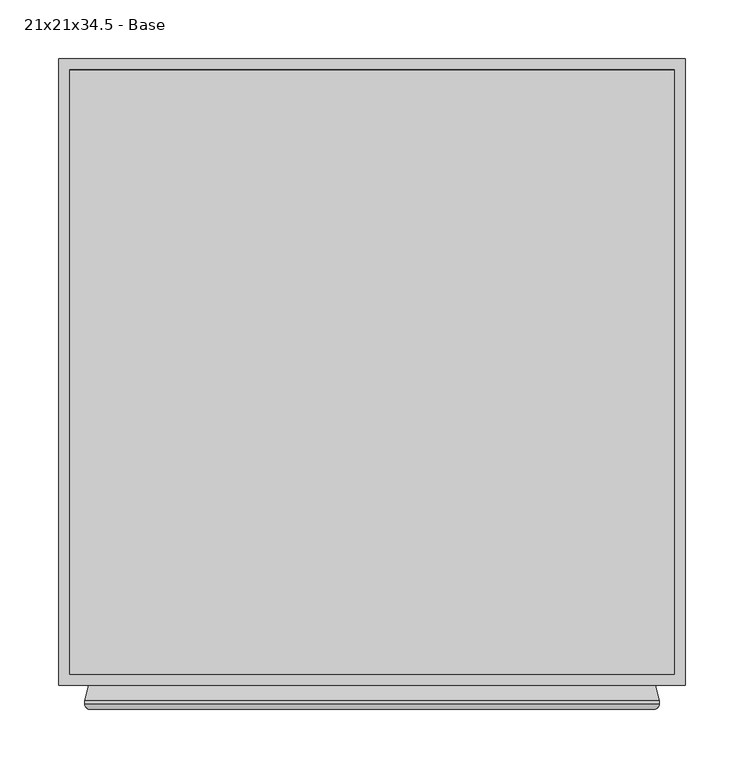
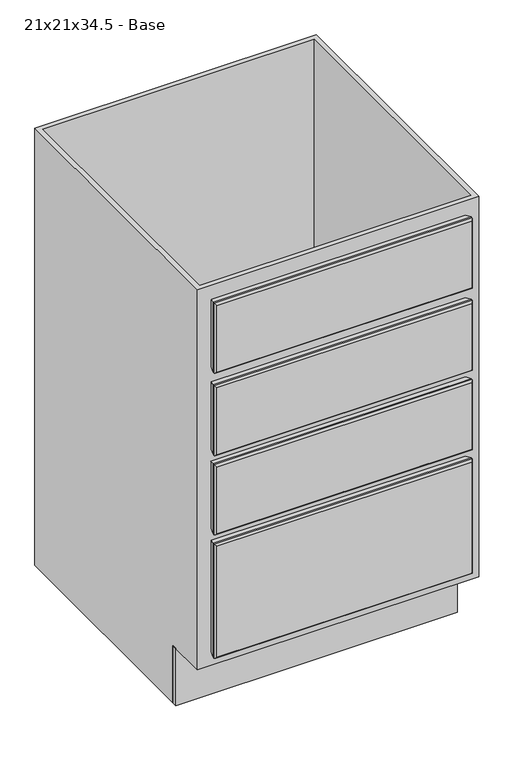
"""IFC4 building model written with IfcOpenShell, lengths in millimetres: furniture geometry, Cabinet-Base-Merillat-Four_Drawer-Marlin : 21x21x34.5 - Base."""

from ifc_helpers import new_model, si_unit, frame, origin, origin_with_axes, place, context, project, spatial, polyline, ellipse_curve, outline, extrude, faceted_brep, source, transform, mapped, element, save
from ifc_brep_helpers import plane_surface, cylinder_surface, advanced_brep


def furniture_21x21x34_5_base_fafdbe70(model_context):
    return source(origin(), model_context, "Body", "SolidModel", [
        advanced_brep(
        [(-222.6408026, -629.92, 365.2035075), (-222.6408026, -629.92, 142.7964925), (260.1162124, -629.92, 142.7964925), (260.1162124, -629.92, 365.2035075), (-222.2320951, -609.6, 143.2052), (-222.2320951, -609.6, 364.7948), (259.7075049, -609.6, 364.7948), (259.7075049, -609.6, 143.2052), (-225.7372951, -625.4496, 368.3), (-225.7372951, -622.681, 368.3), (-225.7372951, -622.681, 139.7), (-225.7372951, -625.4496, 139.7), (263.2127049, -622.681, 139.7), (263.2127049, -625.4496, 139.7), (263.2127049, -622.681, 368.3), (263.2127049, -625.4496, 368.3)],
        [
            (0, 1),
            (1, 2),
            (2, 3),
            (3, 0),
            (4, 5),
            (5, 6),
            (6, 7),
            (7, 4),
            (8, 9),
            (9, 10),
            (10, 11),
            (11, 8),
            (10, 12),
            (12, 13),
            (13, 11),
            (12, 14),
            (14, 15),
            (15, 13),
            (8, 15),
            (14, 9),
            (11, 1, ellipse_curve(frame((-220.9620951, -625.4496, 144.4752), z_axis=(-0.7071067811865475, 0.0, 0.7071067811865475), x_axis=(-0.7071067811865474, 0.0, -0.7071067811865476)), 6.7531526, 4.7752)),
            (0, 8, ellipse_curve(frame((-220.9620951, -625.4496, 363.5248), z_axis=(-0.7071067811865475, 0.0, -0.7071067811865475), x_axis=(0.7071067811865474, 0.0, -0.7071067811865476)), 6.7531526, 4.7752)),
            (4, 10),
            (9, 5),
            (13, 2, ellipse_curve(frame((258.4375049, -625.4496, 144.4752), z_axis=(-0.7071067811865475, 0.0, -0.7071067811865475), x_axis=(0.7071067811865476, 0.0, -0.7071067811865474)), 6.7531526, 4.7752)),
            (7, 12),
            (15, 3, ellipse_curve(frame((258.4375049, -625.4496, 363.5248), z_axis=(0.7071067811865475, 0.0, -0.7071067811865475), x_axis=(0.7071067811865474, 0.0, 0.7071067811865476)), 6.7531526, 4.7752)),
            (6, 14),
        ],
        [
            plane_surface(frame((-225.7372951, -629.92, 368.3), z_axis=(0.0, -1.0, 0.0), x_axis=(0.0, 0.0, -1.0))),
            plane_surface(frame((-225.7372951, -609.6, 368.3), z_axis=(0.0, 1.0, 0.0), x_axis=(0.0, 0.0, 1.0))),
            plane_surface(frame((-225.7372951, -629.92, 368.3), z_axis=(-1.0, 0.0, 0.0), x_axis=(0.0, 1.0, 0.0))),
            plane_surface(frame((-225.7372951, -629.92, 139.7), z_axis=(0.0, 0.0, -1.0), x_axis=(0.0, 1.0, 0.0))),
            plane_surface(frame((263.2127049, -629.92, 139.7), z_axis=(1.0, 0.0, 0.0), x_axis=(0.0, 1.0, 0.0))),
            plane_surface(frame((263.2127049, -629.92, 368.3), z_axis=(0.0, 0.0, 1.0), x_axis=(0.0, 1.0, 0.0))),
            cylinder_surface(frame((-220.9620951, -625.4496, 368.3), z_axis=(0.0, 0.0, -1.0), x_axis=(0.0, 1.0, 0.0)), 4.7752),
            plane_surface(frame((-225.7372951, -622.681, 368.3), z_axis=(-0.9659229350723619, 0.25882983502910506, 0.0), x_axis=(0.0, 0.0, -1.0))),
            cylinder_surface(frame((-225.7372951, -625.4496, 144.4752), z_axis=(1.0, 0.0, 0.0), x_axis=(0.0, 1.0, 0.0)), 4.7752),
            plane_surface(frame((-225.7372951, -622.681, 139.7), z_axis=(0.0, 0.25882983502910506, -0.9659229350723619), x_axis=(1.0, 0.0, 0.0))),
            cylinder_surface(frame((258.4375049, -625.4496, 139.7), z_axis=(0.0, 0.0, 1.0), x_axis=(0.0, 1.0, 0.0)), 4.7752),
            plane_surface(frame((263.2127049, -622.681, 139.7), z_axis=(0.9659229350723619, 0.25882983502910506, 0.0), x_axis=(0.0, 0.0, 1.0))),
            cylinder_surface(frame((263.2127049, -625.4496, 363.5248), z_axis=(-1.0, 0.0, 0.0), x_axis=(0.0, 1.0, 0.0)), 4.7752),
            plane_surface(frame((263.2127049, -622.681, 368.3), z_axis=(0.0, 0.25882983502910506, 0.9659229350723619), x_axis=(-1.0, 0.0, 0.0))),
        ],
        [
            (0, [[1, 2, 3, 4]]),
            (1, [[5, 6, 7, 8]]),
            (2, [[9, 10, 11, 12]]),
            (3, [[-11, 13, 14, 15]]),
            (4, [[-14, 16, 17, 18]]),
            (5, [[-9, 19, -17, 20]]),
            (6, [[21, -1, 22, -12]]),
            (7, [[23, -10, 24, -5]]),
            (8, [[-21, -15, 25, -2]]),
            (9, [[-23, -8, 26, -13]]),
            (10, [[-25, -18, 27, -3]]),
            (11, [[-26, -7, 28, -16]]),
            (12, [[-22, -4, -27, -19]]),
            (13, [[-24, -20, -28, -6]]),
        ],
    ),
        advanced_brep(
        [(-222.6408026, -629.92, 523.9535075), (-222.6408026, -629.92, 390.4464925), (260.1162124, -629.92, 390.4464925), (260.1162124, -629.92, 523.9535075), (-222.2320951, -609.6, 390.8552), (-222.2320951, -609.6, 523.5448), (259.7075049, -609.6, 523.5448), (259.7075049, -609.6, 390.8552), (-225.7372951, -625.4496, 527.05), (-225.7372951, -622.681, 527.05), (-225.7372951, -622.681, 387.35), (-225.7372951, -625.4496, 387.35), (263.2127049, -622.681, 387.35), (263.2127049, -625.4496, 387.35), (263.2127049, -622.681, 527.05), (263.2127049, -625.4496, 527.05)],
        [
            (0, 1),
            (1, 2),
            (2, 3),
            (3, 0),
            (4, 5),
            (5, 6),
            (6, 7),
            (7, 4),
            (8, 9),
            (9, 10),
            (10, 11),
            (11, 8),
            (10, 12),
            (12, 13),
            (13, 11),
            (12, 14),
            (14, 15),
            (15, 13),
            (8, 15),
            (14, 9),
            (11, 1, ellipse_curve(frame((-220.9620951, -625.4496, 392.1252), z_axis=(-0.7071067811865475, 0.0, 0.7071067811865475), x_axis=(-0.7071067811865474, 0.0, -0.7071067811865476)), 6.7531526, 4.7752)),
            (0, 8, ellipse_curve(frame((-220.9620951, -625.4496, 522.2748), z_axis=(-0.7071067811865475, 0.0, -0.7071067811865475), x_axis=(0.7071067811865474, 0.0, -0.7071067811865476)), 6.7531526, 4.7752)),
            (4, 10),
            (9, 5),
            (13, 2, ellipse_curve(frame((258.4375049, -625.4496, 392.1252), z_axis=(-0.7071067811865475, 0.0, -0.7071067811865475), x_axis=(0.7071067811865476, 0.0, -0.7071067811865474)), 6.7531526, 4.7752)),
            (7, 12),
            (15, 3, ellipse_curve(frame((258.4375049, -625.4496, 522.2748), z_axis=(0.7071067811865475, 0.0, -0.7071067811865475), x_axis=(0.7071067811865474, 0.0, 0.7071067811865476)), 6.7531526, 4.7752)),
            (6, 14),
        ],
        [
            plane_surface(frame((-225.7372951, -629.92, 527.05), z_axis=(0.0, -1.0, 0.0), x_axis=(0.0, 0.0, -1.0))),
            plane_surface(frame((-225.7372951, -609.6, 527.05), z_axis=(0.0, 1.0, 0.0), x_axis=(0.0, 0.0, 1.0))),
            plane_surface(frame((-225.7372951, -629.92, 527.05), z_axis=(-1.0, 0.0, 0.0), x_axis=(0.0, 1.0, 0.0))),
            plane_surface(frame((-225.7372951, -629.92, 387.35), z_axis=(0.0, 0.0, -1.0), x_axis=(0.0, 1.0, 0.0))),
            plane_surface(frame((263.2127049, -629.92, 387.35), z_axis=(1.0, 0.0, 0.0), x_axis=(0.0, 1.0, 0.0))),
            plane_surface(frame((263.2127049, -629.92, 527.05), z_axis=(0.0, 0.0, 1.0), x_axis=(0.0, 1.0, 0.0))),
            cylinder_surface(frame((-220.9620951, -625.4496, 527.05), z_axis=(0.0, 0.0, -1.0), x_axis=(0.0, 1.0, 0.0)), 4.7752),
            plane_surface(frame((-225.7372951, -622.681, 527.05), z_axis=(-0.9659229350723619, 0.25882983502910506, 0.0), x_axis=(0.0, 0.0, -1.0))),
            cylinder_surface(frame((-225.7372951, -625.4496, 392.1252), z_axis=(1.0, 0.0, 0.0), x_axis=(0.0, 1.0, 0.0)), 4.7752),
            plane_surface(frame((-225.7372951, -622.681, 387.35), z_axis=(0.0, 0.25882983502910506, -0.9659229350723619), x_axis=(1.0, 0.0, 0.0))),
            cylinder_surface(frame((258.4375049, -625.4496, 387.35), z_axis=(0.0, 0.0, 1.0), x_axis=(0.0, 1.0, 0.0)), 4.7752),
            plane_surface(frame((263.2127049, -622.681, 387.35), z_axis=(0.9659229350723619, 0.25882983502910506, 0.0), x_axis=(0.0, 0.0, 1.0))),
            cylinder_surface(frame((263.2127049, -625.4496, 522.2748), z_axis=(-1.0, 0.0, 0.0), x_axis=(0.0, 1.0, 0.0)), 4.7752),
            plane_surface(frame((263.2127049, -622.681, 527.05), z_axis=(0.0, 0.25882983502910506, 0.9659229350723619), x_axis=(-1.0, 0.0, 0.0))),
        ],
        [
            (0, [[1, 2, 3, 4]]),
            (1, [[5, 6, 7, 8]]),
            (2, [[9, 10, 11, 12]]),
            (3, [[-11, 13, 14, 15]]),
            (4, [[-14, 16, 17, 18]]),
            (5, [[-9, 19, -17, 20]]),
            (6, [[21, -1, 22, -12]]),
            (7, [[23, -10, 24, -5]]),
            (8, [[-21, -15, 25, -2]]),
            (9, [[-23, -8, 26, -13]]),
            (10, [[-25, -18, 27, -3]]),
            (11, [[-26, -7, 28, -16]]),
            (12, [[-22, -4, -27, -19]]),
            (13, [[-24, -20, -28, -6]]),
        ],
    ),
        advanced_brep(
        [(-222.6408026, -629.92, 682.7035075), (-222.6408026, -629.92, 549.1964925), (260.1162124, -629.92, 549.1964925), (260.1162124, -629.92, 682.7035075), (-222.2320951, -609.6, 549.6052), (-222.2320951, -609.6, 682.2948), (259.7075049, -609.6, 682.2948), (259.7075049, -609.6, 549.6052), (-225.7372951, -625.4496, 685.8), (-225.7372951, -622.681, 685.8), (-225.7372951, -622.681, 546.1), (-225.7372951, -625.4496, 546.1), (263.2127049, -622.681, 546.1), (263.2127049, -625.4496, 546.1), (263.2127049, -622.681, 685.8), (263.2127049, -625.4496, 685.8)],
        [
            (0, 1),
            (1, 2),
            (2, 3),
            (3, 0),
            (4, 5),
            (5, 6),
            (6, 7),
            (7, 4),
            (8, 9),
            (9, 10),
            (10, 11),
            (11, 8),
            (10, 12),
            (12, 13),
            (13, 11),
            (12, 14),
            (14, 15),
            (15, 13),
            (8, 15),
            (14, 9),
            (11, 1, ellipse_curve(frame((-220.9620951, -625.4496, 550.8752), z_axis=(-0.7071067811865475, 0.0, 0.7071067811865475), x_axis=(-0.7071067811865474, 0.0, -0.7071067811865476)), 6.7531526, 4.7752)),
            (0, 8, ellipse_curve(frame((-220.9620951, -625.4496, 681.0248), z_axis=(-0.7071067811865475, 0.0, -0.7071067811865475), x_axis=(0.7071067811865474, 0.0, -0.7071067811865476)), 6.7531526, 4.7752)),
            (4, 10),
            (9, 5),
            (13, 2, ellipse_curve(frame((258.4375049, -625.4496, 550.8752), z_axis=(-0.7071067811865475, 0.0, -0.7071067811865475), x_axis=(0.7071067811865476, 0.0, -0.7071067811865474)), 6.7531526, 4.7752)),
            (7, 12),
            (15, 3, ellipse_curve(frame((258.4375049, -625.4496, 681.0248), z_axis=(0.7071067811865475, 0.0, -0.7071067811865475), x_axis=(0.7071067811865474, 0.0, 0.7071067811865476)), 6.7531526, 4.7752)),
            (6, 14),
        ],
        [
            plane_surface(frame((-225.7372951, -629.92, 685.8), z_axis=(0.0, -1.0, 0.0), x_axis=(0.0, 0.0, -1.0))),
            plane_surface(frame((-225.7372951, -609.6, 685.8), z_axis=(0.0, 1.0, 0.0), x_axis=(0.0, 0.0, 1.0))),
            plane_surface(frame((-225.7372951, -629.92, 685.8), z_axis=(-1.0, 0.0, 0.0), x_axis=(0.0, 1.0, 0.0))),
            plane_surface(frame((-225.7372951, -629.92, 546.1), z_axis=(0.0, 0.0, -1.0), x_axis=(0.0, 1.0, 0.0))),
            plane_surface(frame((263.2127049, -629.92, 546.1), z_axis=(1.0, 0.0, 0.0), x_axis=(0.0, 1.0, 0.0))),
            plane_surface(frame((263.2127049, -629.92, 685.8), z_axis=(0.0, 0.0, 1.0), x_axis=(0.0, 1.0, 0.0))),
            cylinder_surface(frame((-220.9620951, -625.4496, 685.8), z_axis=(0.0, 0.0, -1.0), x_axis=(0.0, 1.0, 0.0)), 4.7752),
            plane_surface(frame((-225.7372951, -622.681, 685.8), z_axis=(-0.9659229350723619, 0.25882983502910506, 0.0), x_axis=(0.0, 0.0, -1.0))),
            cylinder_surface(frame((-225.7372951, -625.4496, 550.8752), z_axis=(1.0, 0.0, 0.0), x_axis=(0.0, 1.0, 0.0)), 4.7752),
            plane_surface(frame((-225.7372951, -622.681, 546.1), z_axis=(0.0, 0.25882983502910506, -0.9659229350723619), x_axis=(1.0, 0.0, 0.0))),
            cylinder_surface(frame((258.4375049, -625.4496, 546.1), z_axis=(0.0, 0.0, 1.0), x_axis=(0.0, 1.0, 0.0)), 4.7752),
            plane_surface(frame((263.2127049, -622.681, 546.1), z_axis=(0.9659229350723619, 0.25882983502910506, 0.0), x_axis=(0.0, 0.0, 1.0))),
            cylinder_surface(frame((263.2127049, -625.4496, 681.0248), z_axis=(-1.0, 0.0, 0.0), x_axis=(0.0, 1.0, 0.0)), 4.7752),
            plane_surface(frame((263.2127049, -622.681, 685.8), z_axis=(0.0, 0.25882983502910506, 0.9659229350723619), x_axis=(-1.0, 0.0, 0.0))),
        ],
        [
            (0, [[1, 2, 3, 4]]),
            (1, [[5, 6, 7, 8]]),
            (2, [[9, 10, 11, 12]]),
            (3, [[-11, 13, 14, 15]]),
            (4, [[-14, 16, 17, 18]]),
            (5, [[-9, 19, -17, 20]]),
            (6, [[21, -1, 22, -12]]),
            (7, [[23, -10, 24, -5]]),
            (8, [[-21, -15, 25, -2]]),
            (9, [[-23, -8, 26, -13]]),
            (10, [[-25, -18, 27, -3]]),
            (11, [[-26, -7, 28, -16]]),
            (12, [[-22, -4, -27, -19]]),
            (13, [[-24, -20, -28, -6]]),
        ],
    ),
        advanced_brep(
        [(-222.6408026, -629.92, 847.8035075), (-222.6408026, -629.92, 714.2964925), (260.1162124, -629.92, 714.2964925), (260.1162124, -629.92, 847.8035075), (-222.2320951, -609.6, 714.7052), (-222.2320951, -609.6, 847.3948), (259.7075049, -609.6, 847.3948), (259.7075049, -609.6, 714.7052), (-225.7372951, -625.4496, 850.9), (-225.7372951, -622.681, 850.9), (-225.7372951, -622.681, 711.2), (-225.7372951, -625.4496, 711.2), (263.2127049, -622.681, 711.2), (263.2127049, -625.4496, 711.2), (263.2127049, -622.681, 850.9), (263.2127049, -625.4496, 850.9)],
        [
            (0, 1),
            (1, 2),
            (2, 3),
            (3, 0),
            (4, 5),
            (5, 6),
            (6, 7),
            (7, 4),
            (8, 9),
            (9, 10),
            (10, 11),
            (11, 8),
            (10, 12),
            (12, 13),
            (13, 11),
            (12, 14),
            (14, 15),
            (15, 13),
            (8, 15),
            (14, 9),
            (11, 1, ellipse_curve(frame((-220.9620951, -625.4496, 715.9752), z_axis=(-0.7071067811865475, 0.0, 0.7071067811865475), x_axis=(-0.7071067811865474, 0.0, -0.7071067811865476)), 6.7531526, 4.7752)),
            (0, 8, ellipse_curve(frame((-220.9620951, -625.4496, 846.1248), z_axis=(-0.7071067811865475, 0.0, -0.7071067811865475), x_axis=(0.7071067811865474, 0.0, -0.7071067811865476)), 6.7531526, 4.7752)),
            (4, 10),
            (9, 5),
            (13, 2, ellipse_curve(frame((258.4375049, -625.4496, 715.9752), z_axis=(-0.7071067811865475, 0.0, -0.7071067811865475), x_axis=(0.7071067811865476, 0.0, -0.7071067811865474)), 6.7531526, 4.7752)),
            (7, 12),
            (15, 3, ellipse_curve(frame((258.4375049, -625.4496, 846.1248), z_axis=(0.7071067811865475, 0.0, -0.7071067811865475), x_axis=(0.7071067811865474, 0.0, 0.7071067811865476)), 6.7531526, 4.7752)),
            (6, 14),
        ],
        [
            plane_surface(frame((-225.7372951, -629.92, 850.9), z_axis=(0.0, -1.0, 0.0), x_axis=(0.0, 0.0, -1.0))),
            plane_surface(frame((-225.7372951, -609.6, 850.9), z_axis=(0.0, 1.0, 0.0), x_axis=(0.0, 0.0, 1.0))),
            plane_surface(frame((-225.7372951, -629.92, 850.9), z_axis=(-1.0, 0.0, 0.0), x_axis=(0.0, 1.0, 0.0))),
            plane_surface(frame((-225.7372951, -629.92, 711.2), z_axis=(0.0, 0.0, -1.0), x_axis=(0.0, 1.0, 0.0))),
            plane_surface(frame((263.2127049, -629.92, 711.2), z_axis=(1.0, 0.0, 0.0), x_axis=(0.0, 1.0, 0.0))),
            plane_surface(frame((263.2127049, -629.92, 850.9), z_axis=(0.0, 0.0, 1.0), x_axis=(0.0, 1.0, 0.0))),
            cylinder_surface(frame((-220.9620951, -625.4496, 850.9), z_axis=(0.0, 0.0, -1.0), x_axis=(0.0, 1.0, 0.0)), 4.7752),
            plane_surface(frame((-225.7372951, -622.681, 850.9), z_axis=(-0.9659229350723619, 0.25882983502910506, 0.0), x_axis=(0.0, 0.0, -1.0))),
            cylinder_surface(frame((-225.7372951, -625.4496, 715.9752), z_axis=(1.0, 0.0, 0.0), x_axis=(0.0, 1.0, 0.0)), 4.7752),
            plane_surface(frame((-225.7372951, -622.681, 711.2), z_axis=(0.0, 0.25882983502910506, -0.9659229350723619), x_axis=(1.0, 0.0, 0.0))),
            cylinder_surface(frame((258.4375049, -625.4496, 711.2), z_axis=(0.0, 0.0, 1.0), x_axis=(0.0, 1.0, 0.0)), 4.7752),
            plane_surface(frame((263.2127049, -622.681, 711.2), z_axis=(0.9659229350723619, 0.25882983502910506, 0.0), x_axis=(0.0, 0.0, 1.0))),
            cylinder_surface(frame((263.2127049, -625.4496, 846.1248), z_axis=(-1.0, 0.0, 0.0), x_axis=(0.0, 1.0, 0.0)), 4.7752),
            plane_surface(frame((263.2127049, -622.681, 850.9), z_axis=(0.0, 0.25882983502910506, 0.9659229350723619), x_axis=(-1.0, 0.0, 0.0))),
        ],
        [
            (0, [[1, 2, 3, 4]]),
            (1, [[5, 6, 7, 8]]),
            (2, [[9, 10, 11, 12]]),
            (3, [[-11, 13, 14, 15]]),
            (4, [[-14, 16, 17, 18]]),
            (5, [[-9, 19, -17, 20]]),
            (6, [[21, -1, 22, -12]]),
            (7, [[23, -10, 24, -5]]),
            (8, [[-21, -15, 25, -2]]),
            (9, [[-23, -8, 26, -13]]),
            (10, [[-25, -18, 27, -3]]),
            (11, [[-26, -7, 28, -16]]),
            (12, [[-22, -4, -27, -19]]),
            (13, [[-24, -20, -28, -6]]),
        ],
    ),
        extrude(outline(polyline([(285.4377049, -529.43125), (285.4377049, -538.95625), (-247.9622951, -538.95625), (-247.9622951, -529.43125), (285.4377049, -529.43125)])), origin_with_axes(), (0.0, 0.0, 1.0), 114.3),
        faceted_brep([(285.4377049, -76.2, 0.0), (285.4377049, -529.43125, 0.0), (275.9127049, -529.43125, 0.0), (275.9127049, -85.725, 0.0), (-238.4372951, -85.725, 0.0), (-238.4372951, -529.43125, 0.0), (-247.9622951, -529.43125, 0.0), (-247.9622951, -76.2, 0.0), (-247.9622951, -76.2, 876.3), (285.4377049, -76.2, 876.3), (-247.9622951, -529.43125, 114.3), (-247.9622951, -609.6, 114.3), (-247.9622951, -609.6, 876.3), (285.4377049, -609.6, 876.3), (285.4377049, -609.6, 114.3), (285.4377049, -529.43125, 114.3), (275.9127049, -529.43125, 114.3), (275.9127049, -85.725, 114.3), (275.9127049, -600.075, 876.3), (275.9127049, -85.725, 876.3), (275.9127049, -85.725, 119.0625), (275.9127049, -600.075, 119.0625), (-238.4372951, -85.725, 114.3), (-238.4372951, -529.43125, 114.3), (-238.4372951, -85.725, 876.3), (-238.4372951, -600.075, 876.3), (-238.4372951, -600.075, 119.0625), (-238.4372951, -85.725, 119.0625)], [[[0, 1, 2, 3, 4, 5, 6, 7]], [[0, 7, 8, 9]], [[7, 6, 10, 11, 12, 8]], [[1, 0, 9, 13, 14, 15]], [[3, 2, 16, 17]], [[18, 19, 20, 21]], [[5, 4, 22, 23]], [[24, 25, 26, 27]], [[4, 3, 17, 22]], [[19, 24, 27, 20]], [[9, 8, 12, 13], [19, 18, 25, 24]], [[14, 11, 10, 23, 22, 17, 16, 15]], [[13, 12, 11, 14]], [[25, 18, 21, 26]], [[6, 5, 23, 10]], [[2, 1, 15, 16]], [[21, 20, 27, 26]]]),
    ])


if __name__ == "__main__":
    model = new_model("IFC4")
    model_context = context("Model", 3, world=origin())
    ifc_project = project(units=[si_unit("LENGTHUNIT", "METRE", prefix="MILLI")], contexts=[model_context])
    site = spatial("IfcSite", under=ifc_project)
    building = spatial("IfcBuilding", under=site)
    placement = place(None, origin())
    furniture_21x21x34_5_base_shape = furniture_21x21x34_5_base_fafdbe70(model_context)
    element("IfcFurniture", 1, ObjectType="Cabinet-Base-Merillat-Four_Drawer-Marlin : 21x21x34.5 - Base", at=placement, inside=building, context=model_context, shape_type="MappedRepresentation", body=[
        mapped(furniture_21x21x34_5_base_shape, transform((0.0, 0.0, 0.0), x_axis=(1.0, 0.0, 0.0), y_axis=(0.0, 1.0, 0.0), z_axis=(0.0, 0.0, 1.0))),
    ])
    save(model, "model.ifc")

# Revit data of these elements
# Type "Cabinet-Base-Merillat-Four_Drawer-Marlin : 21x21x34.5 - Base"
#   URL = "http://www.merillat.com"
#   Toe Kick Note = "Toe Kick Covering is not included. To be purchased Separately."
#   Product Line = "Express"
#   Product Page URL = "http://www.merillat.com//our-products/rooms/kitchen/"
#   Product Group = "Base Cabinet"
#   Product Documentation Link = "http://merillatbusiness.com/customer-resources/product-line-resources/merillat-classic/"
#   Model = "BD21-4D"
#   Manufacturer = "Merillat"
#   Finish = "Wood"
#   Description = "Base Four Drawer Cabinet"
#   Construction Type = "Base Four Drawer"
#   Cabinet Construction Note = "3/4 extension sliders on all three drawers when SST or PST construction is chosen"
#   Assembly Code = "C1030410"
#   Top and Bottom Spacing = 0' - 1"
#   Toe Kick Height = 0' - 4 1/2"
#   Toe Kick Depth = 0' - 2 25/32"
#   Cabinet Shell = 0' - 0 3/8"
#   Middle Drawer Spacing = 0' - 0 3/4"
#   Depth = 1' - 9"
#   Height = 2' - 10 1/2"
#   Width = 1' - 9"
#   Deep Cabinet Drawer Height = 0' - 9"
#   Cabinet Drawer Width = 1' - 7 1/4"
#   Cabinet Drawer Height = 0' - 5 1/2"
#   COBie.Type = no
#   Partial Overlay = yes
#   Full Overlay = no
#   Toe Kick Material = Wood - Merillat - Raw Particle Board
#   Door Drawer Material = Wood - Merillat - Pecan(1)
#   Cabinet Drawer Style = element 826866
#   Cabinet Material = Wood - Merillat - Pecan(1)
# Element 1 (IfcFurniture, "Cabinet-Base-Merillat-Four_Drawer-Marlin : 21x21x34.5 - Base")
#   Materials on its faces: "Wood - Merillat - Pecan(1)", "Wood - Merillat - Raw Particle Board"
# Materials
#   "Wood - Merillat - Raw Particle Board": class "Plastic", colour RGB 80 80 80, transparency 0, Description = "Plastic Laminate - Navy", Cost = 0
#   "Wood - Merillat - Pecan(1)": class "Wood", colour RGB 108 67 43, transparency 0, Cost = 0
